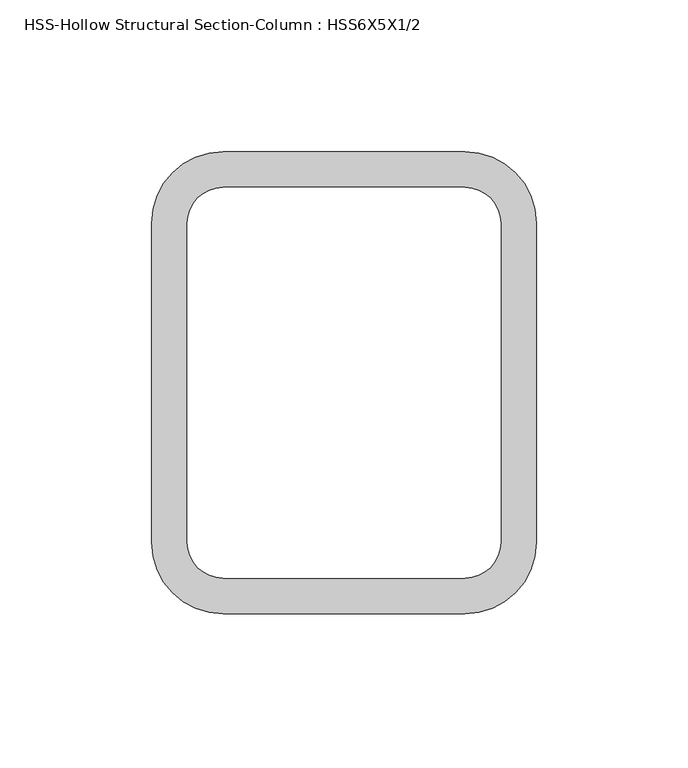
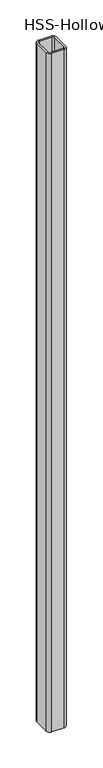
"""IFC4 building model written with IfcOpenShell, lengths in millimetres: column geometry, HSS-Hollow Structural Section-Column : HSS6X5X1/2."""

from ifc_helpers import new_model, si_unit, point, frame, frame_2d, origin, place, context, project, spatial, polyline, circle_curve, trimmed, segment, composite_curve, outline, extrude, source, transform, mapped, element, save


def hss_hollow_structural_section_column_hss6x5x1_2_5e688653(model_context):
    return source(origin(), model_context, "Body", "SweptSolid", [
        extrude(outline(composite_curve([segment(trimmed(circle_curve(frame_2d((39.878, 52.578)), 23.622), [point((39.878, 76.2))], [point((63.5, 52.578))], False, "CARTESIAN"), True, "CONTINUOUS"), segment(polyline([(63.5, 52.578), (63.5, -52.578)]), True, "CONTINUOUS"), segment(trimmed(circle_curve(frame_2d((39.878, -52.578)), 23.622), [point((63.5, -52.578))], [point((39.878, -76.2))], False, "CARTESIAN"), True, "CONTINUOUS"), segment(polyline([(39.878, -76.2), (-39.878, -76.2)]), True, "CONTINUOUS"), segment(trimmed(circle_curve(frame_2d((-39.878, -52.578)), 23.622), [point((-39.878, -76.2))], [point((-63.5, -52.578))], False, "CARTESIAN"), True, "CONTINUOUS"), segment(polyline([(-63.5, -52.578), (-63.5, 52.578)]), True, "CONTINUOUS"), segment(trimmed(circle_curve(frame_2d((-39.878, 52.578)), 23.622), [point((-63.5, 52.578))], [point((-39.878, 76.2))], False, "CARTESIAN"), True, "CONTINUOUS"), segment(polyline([(-39.878, 76.2), (39.878, 76.2)]), True, "CONTINUOUS")], self_intersect=False), holes=[composite_curve([segment(polyline([(39.878, 64.389), (-39.878, 64.389)]), True, "CONTINUOUS"), segment(trimmed(circle_curve(frame_2d((-39.878, 52.578)), 11.811), [point((-39.878, 64.389))], [point((-51.689, 52.578))], True, "CARTESIAN"), True, "CONTINUOUS"), segment(polyline([(-51.689, 52.578), (-51.689, -52.578)]), True, "CONTINUOUS"), segment(trimmed(circle_curve(frame_2d((-39.878, -52.578)), 11.811), [point((-51.689, -52.578))], [point((-39.878, -64.389))], True, "CARTESIAN"), True, "CONTINUOUS"), segment(polyline([(-39.878, -64.389), (39.878, -64.389)]), True, "CONTINUOUS"), segment(trimmed(circle_curve(frame_2d((39.878, -52.578)), 11.811), [point((39.878, -64.389))], [point((51.689, -52.578))], True, "CARTESIAN"), True, "CONTINUOUS"), segment(polyline([(51.689, -52.578), (51.689, 52.578)]), True, "CONTINUOUS"), segment(trimmed(circle_curve(frame_2d((39.878, 52.578)), 11.811), [point((51.689, 52.578))], [point((39.878, 64.389))], True, "CARTESIAN"), True, "CONTINUOUS")], self_intersect=False)]), frame((0.0, 0.0, -304.8), z_axis=(0.0, 0.0, 1.0), x_axis=(1.0, 0.0, 0.0)), (0.0, 0.0, 1.0), 4718.05),
    ])


if __name__ == "__main__":
    model = new_model("IFC4")
    model_context = context("Model", 3, world=origin())
    ifc_project = project(units=[si_unit("LENGTHUNIT", "METRE", prefix="MILLI")], contexts=[model_context])
    site = spatial("IfcSite", under=ifc_project)
    building = spatial("IfcBuilding", under=site)
    placement = place(None, origin())
    hss_hollow_structural_section_column_hss6x5x1_2_shape = hss_hollow_structural_section_column_hss6x5x1_2_5e688653(model_context)
    element("IfcColumn", 1, ObjectType="HSS-Hollow Structural Section-Column : HSS6X5X1/2", at=placement, inside=building, context=model_context, shape_type="MappedRepresentation", body=[
        mapped(hss_hollow_structural_section_column_hss6x5x1_2_shape, transform((0.0, 0.0, 0.0), x_axis=(1.0, 0.0, 0.0), y_axis=(0.0, 1.0, 0.0), z_axis=(0.0, 0.0, 1.0))),
    ])
    save(model, "model.ifc")

# Revit data of these elements
# Type "HSS-Hollow Structural Section-Column : HSS6X5X1/2"
#   Assembly Code = "B10"
#   Shape = "Rect."
#   W = 31.7
#   Ht = 0' - 6"
#   b = 0' - 5"
#   kr = 0' - 0.93"
#   t = 0' - 0.465"
#   A = 0.0611806 SF
#   Structural Material [instance default] = Steel ASTM A500, Grade B, Rectangular and Square
# Element 1 (IfcColumn, "HSS-Hollow Structural Section-Column : HSS6X5X1/2")
#   Structural Material = Metal - Steel - ASTM A992
#   Materials on its faces: "Metal - Steel - ASTM A992"
# Materials
#   "Steel ASTM A500, Grade B, Rectangular and Square": class "Metal", colour RGB 199 199 199, transparency 0, Description = "Carbon steel", Cost = 0
#   "Metal - Steel - ASTM A992": class "Metal", colour RGB 255 128 0, transparency 0
